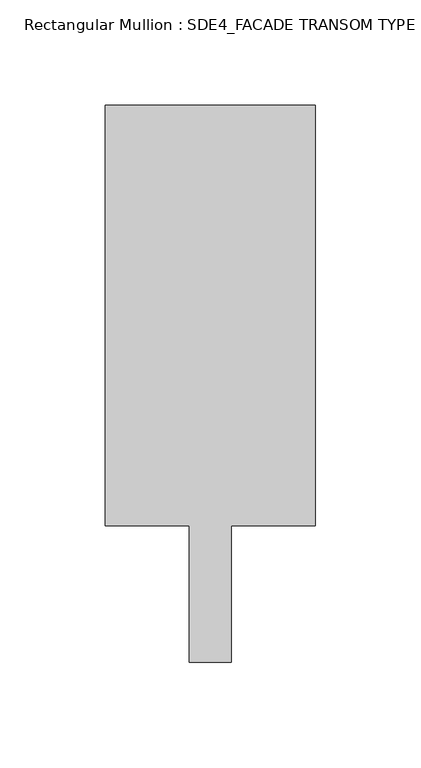
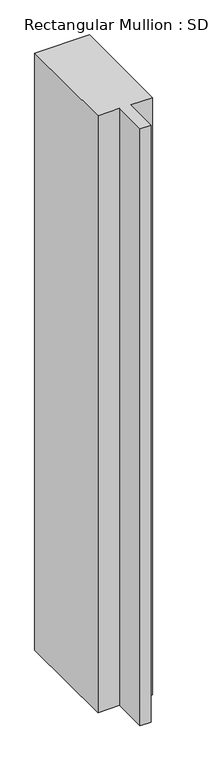
"""IFC4 building model written with IfcOpenShell, lengths in millimetres: member geometry, Rectangular Mullion : SDE4_FACADE TRANSOM TYPE 2."""

from ifc_helpers import new_model, si_unit, frame, origin, place, context, project, spatial, polyline, outline, extrude, source, transform, mapped, element, save


def rectangular_mullion_sde4_facade_transom_type_2_07f1a8ad(model_context):
    return source(origin(), model_context, "Body", "SweptSolid", [
        extrude(outline(polyline([(50.0, 132.5), (50.0, -67.5), (10.0, -67.5), (10.0, -132.5), (-10.0, -132.5), (-10.0, -67.5), (-50.0, -67.5), (-50.0, 132.5), (50.0, 132.5)])), frame((0.0, 0.0, -1155.0), z_axis=(0.0, 0.0, 1.0), x_axis=(1.0, 0.0, 0.0)), (0.0, 0.0, 1.0), 1155.0),
    ])


if __name__ == "__main__":
    model = new_model("IFC4")
    model_context = context("Model", 3, world=origin())
    ifc_project = project(units=[si_unit("LENGTHUNIT", "METRE", prefix="MILLI")], contexts=[model_context])
    site = spatial("IfcSite", under=ifc_project)
    building = spatial("IfcBuilding", under=site)
    placement = place(None, origin())
    rectangular_mullion_sde4_facade_transom_type_2_shape = rectangular_mullion_sde4_facade_transom_type_2_07f1a8ad(model_context)
    element("IfcMember", 1, ObjectType="Rectangular Mullion : SDE4_FACADE TRANSOM TYPE 2", at=placement, inside=building, context=model_context, shape_type="MappedRepresentation", body=[
        mapped(rectangular_mullion_sde4_facade_transom_type_2_shape, transform((0.0, 0.0, 0.0), x_axis=(1.0, 0.0, 0.0), y_axis=(0.0, 1.0, 0.0), z_axis=(0.0, 0.0, 1.0))),
    ])
    save(model, "model.ifc")

# Revit data of these elements
# Type "Rectangular Mullion : SDE4_FACADE TRANSOM TYPE 2"
#   built-in parameter 1007322 = 0.869423 (stored number, unit not read)
#   built-in parameter 1007321 = 0.164042 (stored number, unit not read)
#   built-in parameter 1007320 = 0.164042 (stored number, unit not read)
